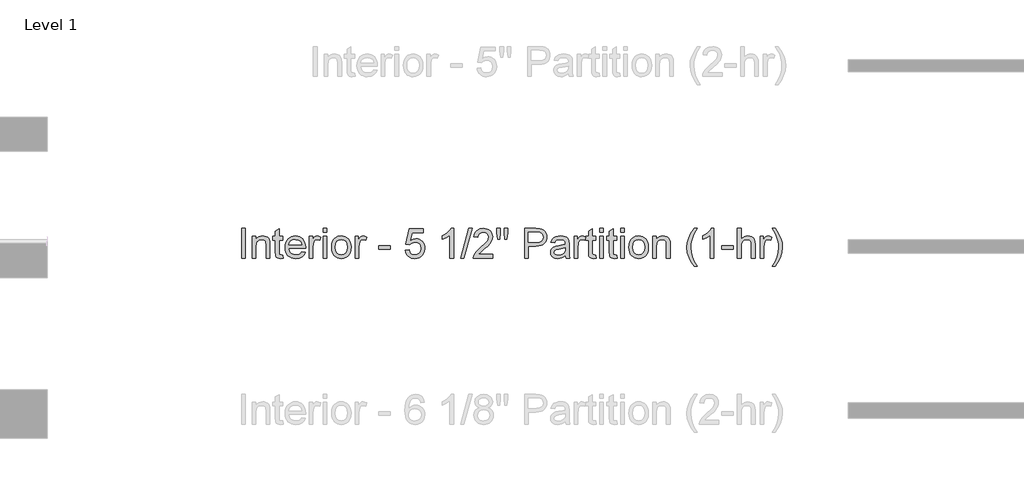
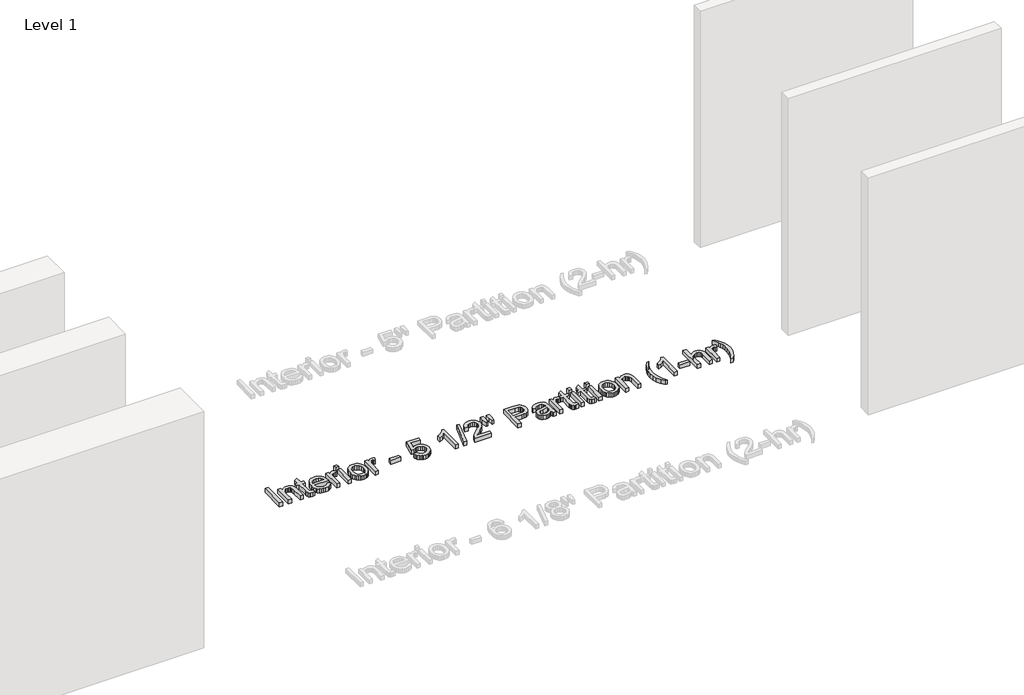
# One storey, part 33 of 42: 1 proxy.
"""IFC4 building model written with IfcOpenShell, lengths in millimetres."""

from ifc_helpers import new_model, si_unit, origin, origin_with_axes, place, context, project, spatial, polyline, outline, extrude, element, save

model = new_model("IFC4")

# Units and contexts
model_context = context("Model", 3, world=origin())
ifc_project = project(units=[si_unit("LENGTHUNIT", "METRE", prefix="MILLI")], contexts=[model_context])

# Site, building, storey
site = spatial("IfcSite", under=ifc_project)
building = spatial("IfcBuilding", under=site)
storey = spatial("IfcBuildingStorey", under=building, Name="Level 1", Elevation=0.0)

# Proxy
placement = place(None, origin())
element("IfcBuildingElementProxy", 1, Name="8\" Arial", ObjectType="8\" Arial", at=placement, inside=storey, context=model_context, shape_type="SweptSolid", body=[
    extrude(outline(polyline([(5266.6577476, 10128.7253326), (5266.6577476, 10433.2924266), (5304.7286344, 10433.2924266), (5304.7286344, 10128.7253326), (5266.6577476, 10128.7253326)])), origin_with_axes(), (0.0, 0.0, 1.0), 50.8),
    extrude(outline(polyline([(5376.111547, 10128.7253326), (5376.111547, 10352.3917923), (5414.1824338, 10352.3917923), (5414.1824338, 10321.161768), (5427.4087209, 10336.9069052), (5443.2932779, 10348.1534318), (5461.8361048, 10354.9013478), (5483.0372016, 10357.1506531), (5501.8031002, 10355.3381963), (5518.9889082, 10349.900826), (5533.3212586, 10341.5170517), (5543.5267844, 10330.8653827), (5554.9406147, 10302.8698966), (5556.9482591, 10266.0630822), (5556.9482591, 10128.7253326), (5518.8773724, 10128.7253326), (5518.8773724, 10260.9324354), (5514.4902975, 10294.6162473), (5508.420891, 10304.6451748), (5498.9868212, 10312.4247969), (5486.8944814, 10317.416024), (5472.8502651, 10319.0797663), (5450.5523996, 10315.343317), (5431.5448402, 10304.133969), (5423.9487874, 10294.983386), (5418.5230354, 10282.4774343), (5414.1824338, 10247.3994249), (5414.1824338, 10128.7253326), (5376.111547, 10128.7253326)])), origin_with_axes(), (0.0, 0.0, 1.0), 50.8),
    extrude(outline(polyline([(5690.1963628, 10160.4758573), (5694.9552236, 10127.6099745), (5666.4764158, 10123.9664717), (5648.2031337, 10125.5465622), (5634.5771767, 10130.2868338), (5624.9479192, 10137.5924287), (5618.6647357, 10146.8684895), (5615.2071259, 10162.7995198), (5614.0545893, 10190.0700231), (5614.0545893, 10314.3209055), (5585.5014242, 10314.3209055), (5585.5014242, 10352.3917923), (5614.0545893, 10352.3917923), (5614.0545893, 10406.746906), (5652.125476, 10429.1284234), (5652.125476, 10352.3917923), (5690.1963628, 10352.3917923), (5690.1963628, 10314.3209055), (5652.125476, 10314.3209055), (5652.125476, 10191.1853811), (5654.1331204, 10171.5550802), (5660.6393755, 10164.6026819), (5673.614707, 10162.0373585), (5690.1963628, 10160.4758573)])), origin_with_axes(), (0.0, 0.0, 1.0), 50.8),
    extrude(outline(polyline([(5884.8635142, 10195.3493844), (5922.190829, 10190.5905235), (5908.7414703, 10162.4649124), (5887.2801232, 10141.4404139), (5858.2901096, 10128.3349572), (5822.2547512, 10123.9664717), (5798.632398, 10125.850962), (5777.5846629, 10131.5044329), (5759.1115459, 10140.9268845), (5743.2130469, 10154.1183166), (5730.4282557, 10170.7115907), (5721.296262, 10190.339568), (5715.8170658, 10213.0022486), (5713.990667, 10238.6996324), (5715.8356551, 10265.2683897), (5721.3706192, 10288.6862606), (5730.5955594, 10308.9532451), (5743.5104757, 10326.0693432), (5759.3671487, 10339.6674163), (5777.4173592, 10349.3803256), (5797.6611071, 10355.2080712), (5820.0983924, 10357.1506531), (5841.8130187, 10355.2127186), (5861.4502907, 10349.3989149), (5879.0102083, 10339.7092422), (5894.4927717, 10326.1437004), (5907.1311722, 10309.0647809), (5916.1586011, 10288.834975), (5921.5750584, 10265.4542827), (5923.3805442, 10238.922704), (5923.1574726, 10228.6614103), (5752.0615538, 10228.6614103), (5758.6514607, 10200.1640131), (5773.9597494, 10179.2138718), (5796.0531326, 10166.3314868), (5822.9983232, 10162.0373585), (5843.2606604, 10164.0264136), (5860.325638, 10169.9935789), (5874.1932559, 10180.3106405), (5884.8635142, 10195.3493844)]), holes=[polyline([(5752.0615538, 10266.7322971), (5885.3096574, 10266.7322971), (5880.1604213, 10286.8459198), (5870.0664313, 10301.2340382), (5847.8708069, 10314.6183343), (5819.949678, 10319.0797663), (5794.2871491, 10315.5199154), (5773.067463, 10304.8403624), (5758.3168533, 10288.1936441), (5752.0615538, 10266.7322971)])]), origin_with_axes(), (0.0, 0.0, 1.0), 50.8),
    extrude(outline(polyline([(5961.4514309, 10128.7253326), (5961.4514309, 10352.3917923), (5994.7634569, 10352.3917923), (5994.7634569, 10319.3028379), (6007.0695736, 10338.4869957), (6018.4090467, 10349.7892902), (6029.7856984, 10355.3103124), (6042.2033509, 10357.1506531), (6061.1644371, 10354.2135437), (6080.4229521, 10345.4022154), (6067.7078707, 10311.2722603), (6054.3235746, 10317.1278898), (6040.9392785, 10319.0797663), (6029.5719214, 10317.202247), (6019.4128689, 10311.5696891), (6011.2056929, 10302.6096464), (6005.6939654, 10290.7496729), (6001.0652296, 10269.4835135), (5999.5223177, 10246.2840669), (5999.5223177, 10128.7253326), (5961.4514309, 10128.7253326)])), origin_with_axes(), (0.0, 0.0, 1.0), 50.8),
    extrude(outline(polyline([(6104.2172563, 10395.2215399), (6104.2172563, 10433.2924266), (6142.288143, 10433.2924266), (6142.288143, 10395.2215399), (6104.2172563, 10395.2215399)])), origin_with_axes(), (0.0, 0.0, 1.0), 50.8),
    extrude(outline(polyline([(6104.2172563, 10128.7253326), (6104.2172563, 10352.3917923), (6142.288143, 10352.3917923), (6142.288143, 10128.7253326), (6104.2172563, 10128.7253326)])), origin_with_axes(), (0.0, 0.0, 1.0), 50.8),
    extrude(outline(polyline([(6189.8767515, 10240.5585624), (6191.9355165, 10269.5253394), (6198.1118115, 10294.4861222), (6208.4056364, 10315.4409108), (6222.8169914, 10332.3897053), (6237.3259402, 10343.2226199), (6253.3406223, 10350.9604161), (6270.8610377, 10355.6030939), (6289.8871864, 10357.1506531), (6310.890772, 10355.2661628), (6329.8820658, 10349.6126919), (6346.8610678, 10340.1902404), (6361.8277781, 10326.9988082), (6374.043272, 10310.4845387), (6382.7686248, 10291.0935749), (6388.0038364, 10268.825917), (6389.748907, 10243.6815648), (6386.6630831, 10205.2203028), (6377.4056117, 10175.942155), (6362.2460374, 10154.0160754), (6341.4539051, 10137.611018), (6316.7580198, 10127.3776083), (6289.8871864, 10123.9664717), (6268.5768774, 10125.843991), (6249.4089853, 10131.476549), (6232.38351, 10140.8641456), (6217.5004516, 10154.0067808), (6205.4150828, 10170.681383), (6196.7826765, 10190.6648807), (6191.6032327, 10213.9572739), (6189.8767515, 10240.5585624)]), holes=[polyline([(6227.9476383, 10240.6329196), (6232.3533024, 10206.1776517), (6245.5702948, 10181.6304809), (6265.460846, 10166.9356391), (6289.8871864, 10162.0373585), (6314.2019911, 10166.963523), (6334.0553637, 10181.7420167), (6347.2723561, 10206.6145003), (6351.6780202, 10241.8226348), (6347.2444721, 10275.2740805), (6333.9438279, 10299.486644), (6314.0625713, 10314.1814857), (6289.8871864, 10319.0797663), (6265.460846, 10314.200075), (6245.5702948, 10299.5610012), (6232.3533024, 10275.0695982), (6227.9476383, 10240.6329196)])]), origin_with_axes(), (0.0, 0.0, 1.0), 50.8),
    extrude(outline(polyline([(6432.5786546, 10128.7253326), (6432.5786546, 10352.3917923), (6465.8906805, 10352.3917923), (6465.8906805, 10319.3028379), (6478.1967972, 10338.4869957), (6489.5362703, 10349.7892902), (6500.912922, 10355.3103124), (6513.3305745, 10357.1506531), (6532.2916607, 10354.2135437), (6551.5501757, 10345.4022154), (6538.8350944, 10311.2722603), (6525.4507983, 10317.1278898), (6512.0665021, 10319.0797663), (6500.6991451, 10317.202247), (6490.5400925, 10311.5696891), (6482.3329165, 10302.6096464), (6476.821189, 10290.7496729), (6472.1924533, 10269.4835135), (6470.6495413, 10246.2840669), (6470.6495413, 10128.7253326), (6432.5786546, 10128.7253326)])), origin_with_axes(), (0.0, 0.0, 1.0), 50.8),
    extrude(outline(polyline([(6675.2805577, 10219.1436886), (6675.2805577, 10257.2145754), (6794.2520788, 10257.2145754), (6794.2520788, 10219.1436886), (6675.2805577, 10219.1436886)])), origin_with_axes(), (0.0, 0.0, 1.0), 50.8),
    extrude(outline(polyline([(6946.5356258, 10209.6259669), (6984.6065126, 10214.3848278), (6991.5960894, 10191.5292832), (7003.7906704, 10175.1614044), (7021.1344874, 10165.3183699), (7043.5717727, 10162.0373585), (7070.8608654, 10166.6010317), (7091.3090956, 10180.2920512), (7104.0799448, 10201.5303267), (7108.3368945, 10228.7357675), (7104.3494897, 10254.3518231), (7092.387275, 10273.9449455), (7072.3573041, 10286.3811873), (7044.1666303, 10290.5266013), (7025.6981606, 10288.8721536), (7010.7430686, 10283.9088104), (6989.3653734, 10266.7322971), (6951.2944867, 10271.4911579), (6984.6065126, 10428.5335658), (7132.1311988, 10428.5335658), (7132.1311988, 10390.462679), (7015.3903937, 10390.462679), (6999.1061667, 10306.5877566), (7026.3023129, 10323.0950552), (7054.79971, 10328.597488), (7073.3402133, 10326.8919197), (7090.3703359, 10321.7752149), (7105.8900779, 10313.2473734), (7119.8994393, 10301.3083954), (7131.4968389, 10286.6879108), (7139.7806958, 10270.1155497), (7144.7510099, 10251.5913121), (7146.4077813, 10231.1151979), (7140.4406159, 10193.0443112), (7132.9816593, 10176.0722801), (7122.5391199, 10160.4758573), (7106.7196254, 10144.5030011), (7088.2604504, 10133.0938181), (7067.1615947, 10126.2483083), (7043.4230583, 10123.9664717), (7023.7764917, 10125.4327028), (7006.030681, 10129.8313959), (6990.1856263, 10137.1625512), (6976.2413275, 10147.4261685), (6964.6392805, 10160.1110422), (6955.8209813, 10174.7059665), (6949.7864297, 10191.2109414), (6946.5356258, 10209.6259669)])), origin_with_axes(), (0.0, 0.0, 1.0), 50.8),
    extrude(outline(polyline([(7441.4571537, 10128.7253326), (7403.3862669, 10128.7253326), (7403.3862669, 10366.0735172), (7367.3230246, 10340.3831043), (7327.2444934, 10321.161768), (7327.2444934, 10357.1506531), (7357.1453827, 10373.4162908), (7383.0495725, 10392.7677522), (7403.4699188, 10413.3461075), (7416.9192774, 10433.2924266), (7441.4571537, 10433.2924266), (7441.4571537, 10128.7253326)])), origin_with_axes(), (0.0, 0.0, 1.0), 50.8),
    extrude(outline(polyline([(7512.8400664, 10128.7253326), (7598.4995616, 10433.2924266), (7632.8525883, 10433.2924266), (7547.1930931, 10128.7253326), (7512.8400664, 10128.7253326)])), origin_with_axes(), (0.0, 0.0, 1.0), 50.8),
    extrude(outline(polyline([(7845.9603255, 10166.7962193), (7845.9603255, 10128.7253326), (7646.08817, 10128.7253326), (7650.177816, 10154.9734244), (7659.5654126, 10175.4867171), (7673.3029055, 10195.386563), (7693.1748674, 10216.2158738), (7720.9658711, 10239.5175616), (7762.0482245, 10276.0083578), (7786.6976365, 10302.9442538), (7799.0223425, 10324.8052708), (7803.1305779, 10346.0714302), (7799.2547088, 10365.1347575), (7787.6271015, 10380.9821359), (7769.7534894, 10391.6616889), (7747.1396058, 10395.2215399), (7723.3917748, 10391.7453407), (7704.9418944, 10381.3167433), (7693.0354476, 10364.7536769), (7688.9179176, 10342.8740706), (7650.8470309, 10347.6329314), (7654.1210713, 10367.286469), (7660.0766184, 10384.4583351), (7668.713672, 10399.1485295), (7680.0322321, 10411.3570524), (7693.7720486, 10420.9537786), (7709.6728713, 10427.8085831), (7747.957535, 10433.2924266), (7768.3616156, 10431.768104), (7786.5210382, 10427.1951362), (7802.4358028, 10419.5735231), (7816.1059094, 10408.9032648), (7827.0852148, 10395.9744065), (7834.9275758, 10381.5769935), (7839.6329924, 10365.7110258), (7841.2014646, 10348.3765034), (7839.5098383, 10330.1682839), (7834.4349594, 10312.2760825), (7825.4284434, 10294.0771576), (7811.9419062, 10274.9487677), (7790.4433805, 10252.1118125), (7757.4008995, 10222.7871914), (7713.6045082, 10186.1662701), (7696.4279949, 10166.7962193), (7845.9603255, 10166.7962193)])), origin_with_axes(), (0.0, 0.0, 1.0), 50.8),
    extrude(outline(polyline([(7969.2445643, 10323.8386272), (7960.1729858, 10382.6551729), (7960.1729858, 10433.2924266), (7998.2438725, 10433.2924266), (7998.2438725, 10382.6551729), (7989.3210084, 10323.8386272), (7969.2445643, 10323.8386272)])), origin_with_axes(), (0.0, 0.0, 1.0), 50.8),
    extrude(outline(polyline([(7893.3258623, 10323.8386272), (7884.0312122, 10382.6551729), (7884.0312122, 10433.2924266), (7922.102099, 10433.2924266), (7922.102099, 10382.6551729), (7913.7740925, 10323.8386272), (7893.3258623, 10323.8386272)])), origin_with_axes(), (0.0, 0.0, 1.0), 50.8),
    extrude(outline(polyline([(8169.5628629, 10128.7253326), (8169.5628629, 10433.2924266), (8282.4370936, 10433.2924266), (8327.9437004, 10430.3924958), (8348.2339216, 10424.9737148), (8364.9364078, 10416.1530919), (8378.3857665, 10403.530957), (8388.916605, 10386.7076404), (8395.7202889, 10366.8635624), (8397.9881835, 10345.1791438), (8396.4568899, 10326.4829551), (8391.8630091, 10309.2832052), (8384.2065411, 10293.5798938), (8373.4874859, 10279.3730212), (8358.7717311, 10267.5966995), (8339.1251645, 10259.1850412), (8314.547786, 10254.1380462), (8285.0395956, 10252.4557145), (8207.6337497, 10252.4557145), (8207.6337497, 10128.7253326), (8169.5628629, 10128.7253326)]), holes=[polyline([(8207.6337497, 10290.5266013), (8287.2703116, 10290.5266013), (8321.0284808, 10294.0213897), (8343.335641, 10304.505755), (8355.7718828, 10321.3290717), (8359.9172967, 10343.8407142), (8357.4728038, 10360.9428703), (8350.1393248, 10375.3681673), (8338.8277357, 10386.2243186), (8324.448912, 10392.6190378), (8286.3780252, 10395.2215399), (8207.6337497, 10395.2215399), (8207.6337497, 10290.5266013)])]), origin_with_axes(), (0.0, 0.0, 1.0), 50.8),
    extrude(outline(polyline([(8588.3426173, 10157.2784976), (8570.1529871, 10141.6820748), (8551.4242671, 10131.476549), (8531.7289036, 10125.843991), (8510.6393426, 10123.9664717), (8478.8237553, 10128.4836716), (8455.3547638, 10142.0352715), (8440.8829936, 10162.6136268), (8436.0590702, 10188.2110931), (8437.8808217, 10203.993409), (8443.3460759, 10218.3257594), (8451.7763235, 10230.5946975), (8462.4930551, 10240.1867764), (8489.1501115, 10252.6787861), (8522.0903515, 10258.4042906), (8561.016346, 10264.4272238), (8588.1195457, 10271.4911579), (8588.3426173, 10279.9678788), (8585.721526, 10296.9584991), (8577.858252, 10308.0749006), (8560.272774, 10316.3285499), (8535.7720764, 10319.0797663), (8513.0931302, 10317.2487203), (8497.2550464, 10311.7555821), (8486.454663, 10301.5965295), (8478.8888179, 10285.7677404), (8440.8179311, 10290.5266013), (8447.4264273, 10311.3466175), (8457.288051, 10327.7052016), (8471.3229727, 10340.2158006), (8490.4513626, 10349.4918614), (8513.8459968, 10355.2359552), (8540.6796516, 10357.1506531), (8566.4165377, 10355.4590268), (8586.8182947, 10350.3841478), (8602.2009406, 10342.7532401), (8612.8804935, 10333.3935275), (8619.9630169, 10321.8216881), (8624.554574, 10307.5544002), (8626.413504, 10274.2423743), (8626.413504, 10226.8768375), (8628.3467913, 10160.7361075), (8635.9312257, 10128.7253326), (8597.860339, 10128.7253326), (8591.7630485, 10141.9609143), (8588.3426173, 10157.2784976)]), holes=[polyline([(8588.3426173, 10233.4202711), (8526.9235695, 10221.7461906), (8494.1692226, 10215.574543), (8479.3349611, 10205.5363209), (8474.129957, 10190.8879523), (8476.9648253, 10179.5670685), (8485.4694301, 10170.2910077), (8499.4578785, 10164.1007708), (8518.7442774, 10162.0373585), (8539.1925076, 10164.3145477), (8557.2613074, 10171.1461156), (8571.9096759, 10181.2122216), (8582.0966124, 10193.1930256), (8586.6138124, 10205.5363209), (8588.1195457, 10222.638477), (8588.3426173, 10233.4202711)])]), origin_with_axes(), (0.0, 0.0, 1.0), 50.8),
    extrude(outline(polyline([(8678.7609733, 10128.7253326), (8678.7609733, 10352.3917923), (8712.0729992, 10352.3917923), (8712.0729992, 10319.3028379), (8724.379116, 10338.4869957), (8735.7185891, 10349.7892902), (8747.0952408, 10355.3103124), (8759.5128933, 10357.1506531), (8778.4739795, 10354.2135437), (8797.7324945, 10345.4022154), (8785.0174131, 10311.2722603), (8771.633117, 10317.1278898), (8758.2488209, 10319.0797663), (8746.8814638, 10317.202247), (8736.7224113, 10311.5696891), (8728.5152353, 10302.6096464), (8723.0035078, 10290.7496729), (8718.374772, 10269.4835135), (8716.8318601, 10246.2840669), (8716.8318601, 10128.7253326), (8678.7609733, 10128.7253326)])), origin_with_axes(), (0.0, 0.0, 1.0), 50.8),
    extrude(outline(polyline([(8902.427433, 10160.4758573), (8907.1862939, 10127.6099745), (8878.707486, 10123.9664717), (8860.4342039, 10125.5465622), (8846.8082469, 10130.2868338), (8837.1789894, 10137.5924287), (8830.895806, 10146.8684895), (8827.4381961, 10162.7995198), (8826.2856595, 10190.0700231), (8826.2856595, 10314.3209055), (8797.7324945, 10314.3209055), (8797.7324945, 10352.3917923), (8826.2856595, 10352.3917923), (8826.2856595, 10406.746906), (8864.3565463, 10429.1284234), (8864.3565463, 10352.3917923), (8902.427433, 10352.3917923), (8902.427433, 10314.3209055), (8864.3565463, 10314.3209055), (8864.3565463, 10191.1853811), (8866.3641907, 10171.5550802), (8872.8704458, 10164.6026819), (8885.8457773, 10162.0373585), (8902.427433, 10160.4758573)])), origin_with_axes(), (0.0, 0.0, 1.0), 50.8),
    extrude(outline(polyline([(8940.4983198, 10395.2215399), (8940.4983198, 10433.2924266), (8978.5692066, 10433.2924266), (8978.5692066, 10395.2215399), (8940.4983198, 10395.2215399)])), origin_with_axes(), (0.0, 0.0, 1.0), 50.8),
    extrude(outline(polyline([(8940.4983198, 10128.7253326), (8940.4983198, 10352.3917923), (8978.5692066, 10352.3917923), (8978.5692066, 10128.7253326), (8940.4983198, 10128.7253326)])), origin_with_axes(), (0.0, 0.0, 1.0), 50.8),
    extrude(outline(polyline([(9116.5761711, 10160.4758573), (9121.3350319, 10127.6099745), (9092.856224, 10123.9664717), (9074.582942, 10125.5465622), (9060.9569849, 10130.2868338), (9051.3277274, 10137.5924287), (9045.044544, 10146.8684895), (9041.5869342, 10162.7995198), (9040.4343975, 10190.0700231), (9040.4343975, 10314.3209055), (9011.8812325, 10314.3209055), (9011.8812325, 10352.3917923), (9040.4343975, 10352.3917923), (9040.4343975, 10406.746906), (9078.5052843, 10429.1284234), (9078.5052843, 10352.3917923), (9116.5761711, 10352.3917923), (9116.5761711, 10314.3209055), (9078.5052843, 10314.3209055), (9078.5052843, 10191.1853811), (9080.5129287, 10171.5550802), (9087.0191838, 10164.6026819), (9099.9945153, 10162.0373585), (9116.5761711, 10160.4758573)])), origin_with_axes(), (0.0, 0.0, 1.0), 50.8),
    extrude(outline(polyline([(9154.6470578, 10395.2215399), (9154.6470578, 10433.2924266), (9192.7179446, 10433.2924266), (9192.7179446, 10395.2215399), (9154.6470578, 10395.2215399)])), origin_with_axes(), (0.0, 0.0, 1.0), 50.8),
    extrude(outline(polyline([(9154.6470578, 10128.7253326), (9154.6470578, 10352.3917923), (9192.7179446, 10352.3917923), (9192.7179446, 10128.7253326), (9154.6470578, 10128.7253326)])), origin_with_axes(), (0.0, 0.0, 1.0), 50.8),
    extrude(outline(polyline([(9240.306553, 10240.5585624), (9242.365318, 10269.5253394), (9248.541613, 10294.4861222), (9258.835438, 10315.4409108), (9273.2467929, 10332.3897053), (9287.7557417, 10343.2226199), (9303.7704238, 10350.9604161), (9321.2908392, 10355.6030939), (9340.316988, 10357.1506531), (9361.3205735, 10355.2661628), (9380.3118673, 10349.6126919), (9397.2908693, 10340.1902404), (9412.2575796, 10326.9988082), (9424.4730735, 10310.4845387), (9433.1984263, 10291.0935749), (9438.433638, 10268.825917), (9440.1787085, 10243.6815648), (9437.0928847, 10205.2203028), (9427.8354132, 10175.942155), (9412.6758389, 10154.0160754), (9391.8837066, 10137.611018), (9367.1878214, 10127.3776083), (9340.316988, 10123.9664717), (9319.006679, 10125.843991), (9299.8387868, 10131.476549), (9282.8133115, 10140.8641456), (9267.9302531, 10154.0067808), (9255.8448843, 10170.681383), (9247.212478, 10190.6648807), (9242.0330343, 10213.9572739), (9240.306553, 10240.5585624)]), holes=[polyline([(9278.3774398, 10240.6329196), (9282.7831039, 10206.1776517), (9296.0000963, 10181.6304809), (9315.8906475, 10166.9356391), (9340.316988, 10162.0373585), (9364.6317926, 10166.963523), (9384.4851652, 10181.7420167), (9397.7021576, 10206.6145003), (9402.1078217, 10241.8226348), (9397.6742737, 10275.2740805), (9384.3736294, 10299.486644), (9364.4923728, 10314.1814857), (9340.316988, 10319.0797663), (9315.8906475, 10314.200075), (9296.0000963, 10299.5610012), (9282.7831039, 10275.0695982), (9278.3774398, 10240.6329196)])]), origin_with_axes(), (0.0, 0.0, 1.0), 50.8),
    extrude(outline(polyline([(9483.0084561, 10128.7253326), (9483.0084561, 10352.3917923), (9521.0793429, 10352.3917923), (9521.0793429, 10321.161768), (9534.3056299, 10336.9069052), (9550.1901869, 10348.1534318), (9568.7330139, 10354.9013478), (9589.9341107, 10357.1506531), (9608.7000092, 10355.3381963), (9625.8858173, 10349.900826), (9640.2181677, 10341.5170517), (9650.4236935, 10330.8653827), (9661.8375238, 10302.8698966), (9663.8451682, 10266.0630822), (9663.8451682, 10128.7253326), (9625.7742815, 10128.7253326), (9625.7742815, 10260.9324354), (9621.3872066, 10294.6162473), (9615.3178001, 10304.6451748), (9605.8837303, 10312.4247969), (9593.7913905, 10317.416024), (9579.7471742, 10319.0797663), (9557.4493087, 10315.343317), (9538.4417492, 10304.133969), (9530.8456964, 10294.983386), (9525.4199445, 10282.4774343), (9521.0793429, 10247.3994249), (9521.0793429, 10128.7253326), (9483.0084561, 10128.7253326)])), origin_with_axes(), (0.0, 0.0, 1.0), 50.8),
    extrude(outline(polyline([(9911.3059321, 10043.0658373), (9881.8047128, 10084.4642088), (9857.2482472, 10132.3688354), (9840.6851808, 10184.4560545), (9835.1641586, 10238.4022036), (9839.2909833, 10285.7119725), (9851.6714572, 10330.9769185), (9876.246512, 10382.2462083), (9911.3059321, 10433.2924266), (9939.8590972, 10433.2924266), (9904.2419981, 10372.9887369), (9882.8271243, 10314.5439771), (9875.6330651, 10276.454501), (9873.2350454, 10238.179132), (9877.3990486, 10189.3729244), (9889.8910583, 10140.5853061), (9910.7110745, 10091.8162771), (9939.8590972, 10043.0658373), (9911.3059321, 10043.0658373)])), origin_with_axes(), (0.0, 0.0, 1.0), 50.8),
    extrude(outline(polyline([(10111.1780876, 10128.7253326), (10073.1072009, 10128.7253326), (10073.1072009, 10366.0735172), (10037.0439585, 10340.3831043), (9996.9654273, 10321.161768), (9996.9654273, 10357.1506531), (10026.8663167, 10373.4162908), (10052.7705065, 10392.7677522), (10073.1908527, 10413.3461075), (10086.6402114, 10433.2924266), (10111.1780876, 10433.2924266), (10111.1780876, 10128.7253326)])), origin_with_axes(), (0.0, 0.0, 1.0), 50.8),
    extrude(outline(polyline([(10192.078722, 10219.1436886), (10192.078722, 10257.2145754), (10311.0502431, 10257.2145754), (10311.0502431, 10219.1436886), (10192.078722, 10219.1436886)])), origin_with_axes(), (0.0, 0.0, 1.0), 50.8),
    extrude(outline(polyline([(10353.8799907, 10128.7253326), (10353.8799907, 10433.2924266), (10391.9508775, 10433.2924266), (10391.9508775, 10321.3104824), (10405.9346785, 10336.9905571), (10421.6379898, 10348.1906104), (10439.0608114, 10354.9106424), (10458.2031433, 10357.1506531), (10481.1981076, 10354.7061601), (10500.9585337, 10347.3726812), (10516.5177779, 10335.7264847), (10526.9091967, 10320.3438388), (10532.7648263, 10299.2078045), (10534.7167028, 10270.3014427), (10534.7167028, 10128.7253326), (10496.6458161, 10128.7253326), (10496.6458161, 10266.360511), (10493.6157601, 10290.1919939), (10484.5255923, 10306.5133994), (10469.8772238, 10315.9381746), (10450.1725656, 10319.0797663), (10434.0835263, 10316.9605861), (10418.9797199, 10310.6030455), (10406.4691209, 10300.6205913), (10398.1597037, 10287.6266704), (10393.503084, 10270.3572106), (10391.9508775, 10247.5481393), (10391.9508775, 10128.7253326), (10353.8799907, 10128.7253326)])), origin_with_axes(), (0.0, 0.0, 1.0), 50.8),
    extrude(outline(polyline([(10587.0641721, 10128.7253326), (10587.0641721, 10352.3917923), (10620.376198, 10352.3917923), (10620.376198, 10319.3028379), (10632.6823147, 10338.4869957), (10644.0217878, 10349.7892902), (10655.3984395, 10355.3103124), (10667.8160921, 10357.1506531), (10686.7771782, 10354.2135437), (10706.0356932, 10345.4022154), (10693.3206119, 10311.2722603), (10679.9363158, 10317.1278898), (10666.5520197, 10319.0797663), (10655.1846626, 10317.202247), (10645.0256101, 10311.5696891), (10636.818434, 10302.6096464), (10631.3067065, 10290.7496729), (10626.6779708, 10269.4835135), (10625.1350589, 10246.2840669), (10625.1350589, 10128.7253326), (10587.0641721, 10128.7253326)])), origin_with_axes(), (0.0, 0.0, 1.0), 50.8),
    extrude(outline(polyline([(10739.3477191, 10043.0658373), (10710.7945541, 10043.0658373), (10739.9425767, 10091.8162771), (10760.7625929, 10140.5853061), (10773.2546027, 10189.3729244), (10777.4186059, 10238.179132), (10775.0205862, 10276.1756615), (10767.826527, 10313.8747623), (10758.7363592, 10343.7477677), (10746.6347248, 10372.3938792), (10710.7945541, 10433.2924266), (10739.3477191, 10433.2924266), (10774.4071393, 10382.2462083), (10798.9821941, 10330.9769185), (10811.362668, 10285.7119725), (10815.4894927, 10238.4022036), (10809.9405866, 10184.4560545), (10793.2938682, 10132.3688354), (10768.7095188, 10084.4642088), (10739.3477191, 10043.0658373)])), origin_with_axes(), (0.0, 0.0, 1.0), 50.8),
])

save(model, "model.ifc")

# Revit data of these elements
# Element 1 (IfcBuildingElementProxy, "8\" Arial")
#   Phase Created = New Construction
